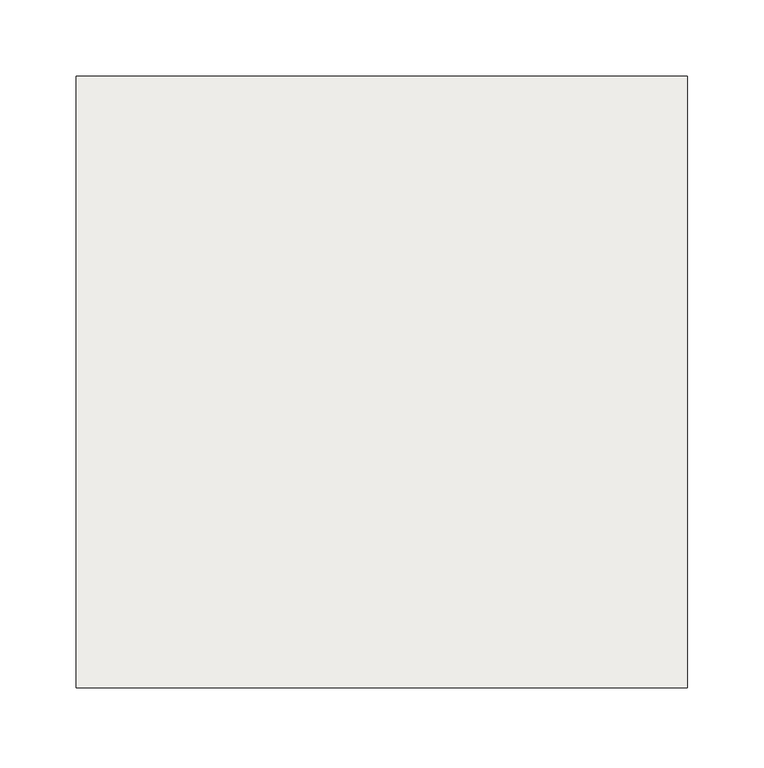
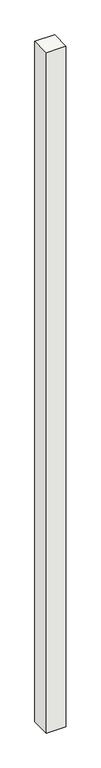
"""IFC4 building model written with IfcOpenShell, lengths in millimetres: footing geometry, NLRS_17_SFO_TLB_funderingspaal geheid beton prefab-AV-MMBPC_gen_rsf : heipaal beton prefab_gen__bxh 400x400."""

from ifc_helpers import new_model, si_unit, frame, origin, place, context, project, spatial, polyline, outline, extrude, source, transform, mapped, element, save


def footing_2462c6b3(model_context):
    return source(origin(), model_context, "Body", "SweptSolid", [
        extrude(outline(polyline([(200.0, -200.0), (-200.0, -200.0), (-200.0, 200.0), (200.0, 200.0), (200.0, -200.0)])), frame((0.0, 0.0, -20000.0), z_axis=(0.0, 0.0, 1.0), x_axis=(1.0, 0.0, 0.0)), (0.0, 0.0, 1.0), 14620.0),
    ])


if __name__ == "__main__":
    model = new_model("IFC4")
    model_context = context("Model", 3, world=origin())
    ifc_project = project(units=[si_unit("LENGTHUNIT", "METRE", prefix="MILLI")], contexts=[model_context])
    site = spatial("IfcSite", under=ifc_project)
    building = spatial("IfcBuilding", under=site)
    placement = place(None, origin())
    footing_shape = footing_2462c6b3(model_context)
    element("IfcFooting", 1, ObjectType="NLRS_17_SFO_TLB_funderingspaal geheid beton prefab-AV-MMBPC_gen_rsf : heipaal beton prefab_gen__bxh 400x400", at=placement, inside=building, context=model_context, shape_type="MappedRepresentation", body=[
        mapped(footing_shape, transform((0.0, 0.0, 0.0), x_axis=(1.0, 0.0, 0.0), y_axis=(0.0, 1.0, 0.0), z_axis=(0.0, 0.0, 1.0))),
    ])
    save(model, "model.ifc")

# Revit data of these elements
# Type "NLRS_17_SFO_TLB_funderingspaal geheid beton prefab-AV-MMBPC_gen_rsf : heipaal beton prefab_gen__bxh 400x400"
#   IfcExportAs = "IfcPile"
#   Type Comments = "prefab heipaal 400x400"
#   Model = " "
#   Manufacturer = " "
#   Description = "prefab heipaal 400x400"
#   Assembly Code = "17.21"
#   Width = 400 mm
#   Slanted Angle [instance default] = 0.00°
#   NLRS_S_draagvermogen_trek [instance default] = 0.00 kN
#   NLRS_S_draagvermogen_druk [instance default] = 0.00 kN
#   NLRS_C_lengte [instance default] = 1660 mm
#   NLRS_C_hoogte = 400 mm
#   NLRS_C_breedte = 400 mm
#   Height [instance default] = 1660 mm
#   Length [instance default] = 1660 mm
#   Angle [instance default] = 0.00°
#   Slanted [instance default] = 0
#   Structural Material = NLRS_f2_beton prefab_gen_rsf
#   Keynote = ""
# Element 1 (IfcFooting, "NLRS_17_SFO_TLB_funderingspaal geheid beton prefab-AV-MMBPC_gen_rsf : heipaal beton prefab_gen__bxh 400x400")
#   NLRS_C_lengte = 14620 mm
#   Height = 14620 mm
#   Length = 14620 mm
#   Materials on its faces: "NLRS_f2_beton prefab_gen_rsf"
# Materials
#   "NLRS_f2_beton prefab_gen_rsf": class "F - Niet gebakken kunststeen", colour RGB 129 133 118, transparency 0, Keynote = "f2", Manufacturer = "Revit Standards Foundation", URL = "www.revitstandards.org", Description = "beton prefab", Cost = 0
